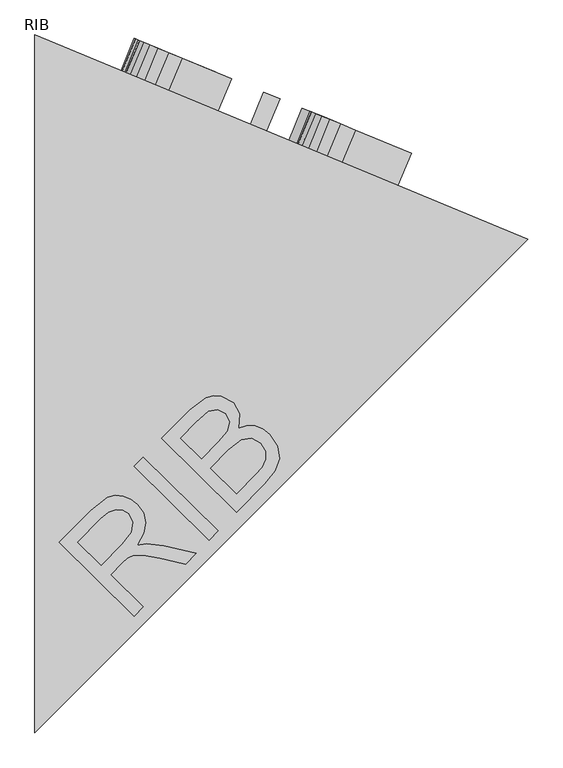
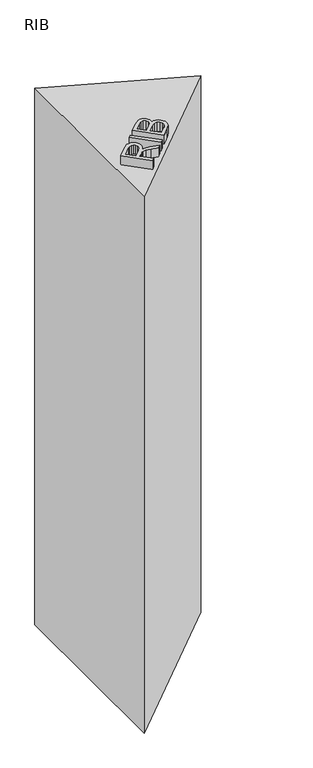
"""IFC4 building model written with IfcOpenShell, lengths in millimetres: geographic element geometry, NO_Origo : RIB."""

from ifc_helpers import new_model, si_unit, frame, origin, origin_with_axes, place, context, project, spatial, polyline, outline, extrude, source, transform, mapped, element, save


def rib_79407f03(model_context):
    return source(origin(), model_context, "Body", "SweptSolid", [
        extrude(outline(polyline([(0.0, 1000.0), (707.1067812, 707.1067812), (0.0, 0.0), (0.0, 1000.0)])), origin_with_axes(), (0.0, 0.0, 1.0), 3000.0),
        extrude(outline(polyline([(25.1140775, 0.0), (25.1140775, -200.9126203), (-61.4608186, -200.9126203), (-84.7293549, -199.5575883), (-101.658058, -195.4924922), (-114.0311558, -187.9876995), (-123.6328759, -176.3135776), (-129.7948993, -161.837421), (-131.8489071, -145.9265248), (-128.4459986, -126.1344734), (-118.2372733, -109.7269364), (-100.9161627, -97.6971952), (-76.1760985, -91.0385311), (-90.4499198, -80.2963768), (-110.806057, -54.4465353), (-144.307844, 0.0), (-115.1225391, 0.0), (-88.9783919, -41.6442419), (-70.0937828, -69.210866), (-56.8255055, -82.2338887), (-44.8816034, -87.0163546), (-30.3134764, -87.8992714), (0.0, -87.8992714), (0.0, 0.0), (25.1140775, 0.0)]), holes=[polyline([(0.0, -113.0133489), (-56.2123689, -113.0133489), (-84.882639, -116.5695415), (-94.3126808, -121.1925919), (-101.1675487, -127.9493579), (-106.7348295, -144.994557), (-104.0799478, -157.2450275), (-96.1153027, -167.1165277), (-82.4116983, -173.628039), (-62.5399392, -175.7985428), (0.0, -175.7985428), (0.0, -113.0133489)])]), frame((497.5715471, 793.899117, 2400.0), z_axis=(0.38268343236508784, 0.9238795325112875, 0.0), x_axis=(0.9238795325112875, -0.38268343236508784, 0.0)), (0.0, 0.0, 1.0), 50.0),
        extrude(outline(polyline([(328.1863632, 918.1803674), (351.3887454, 908.569626), (332.2545738, 862.3756494), (309.0521916, 871.9863908), (328.1863632, 918.1803674)])), frame((0.0, 0.0, 2400.0), z_axis=(0.0, 0.0, 1.0), x_axis=(1.0, 0.0, 0.0)), (0.0, 0.0, 1.0), 200.9126203),
        extrude(outline(polyline([(76.0779965, 0.0), (76.0779965, -200.9126203), (-0.5886112, -200.9126203), (-21.6743809, -199.434961), (-38.1371002, -195.0019829), (-50.7554526, -187.5033216), (-60.3081217, -176.8286123), (-66.3229924, -164.2715736), (-68.3279493, -151.1259236), (-66.6418234, -139.0287373), (-61.583446, -127.6550523), (-53.1160287, -117.7038444), (-41.2027834, -109.8740892), (-55.4336854, -102.4428729), (-65.948979, -91.1366329), (-72.4420962, -76.703396), (-74.6064686, -59.8911888), (-68.6958312, -32.8886504), (-54.0541278, -13.6606848), (-32.2019373, -3.4580908), (0.0, 0.0), (76.0779965, 0.0)]), holes=[polyline([(50.9639191, -119.2918683), (5.101297, -119.2918683), (-21.6805123, -121.4501093), (-37.7937437, -130.7452611), (-43.2138717, -147.1037471), (-38.1616256, -163.4867587), (-23.6916005, -173.1743179), (8.5839132, -175.7985428), (50.9639191, -175.7985428), (50.9639191, -119.2918683)]), polyline([(50.9639191, -25.1140775), (-0.5395603, -25.1140775), (-19.1789147, -26.0950962), (-34.9487895, -31.5642752), (-45.3966382, -42.7233624), (-49.4923911, -59.6459342), (-44.6853997, -79.1682054), (-38.3884862, -86.2254083), (-29.1117286, -90.8178019), (1.9129864, -94.1777908), (50.9639191, -94.1777908), (50.9639191, -25.1140775)])]), frame((192.3605232, 920.3216624, 2400.0), z_axis=(0.38268343236508784, 0.9238795325112875, 0.0), x_axis=(0.9238795325112875, -0.38268343236508784, 0.0)), (0.0, 0.0, 1.0), 50.0),
        extrude(outline(polyline([(142.0846737, 166.9156415), (34.8288922, 272.7551681), (80.4360125, 318.9725642), (104.5051668, 337.5762862), (115.0296187, 340.2280985), (126.319893, 339.2040535), (137.2940026, 334.8676564), (146.8699607, 327.5824121), (155.6431762, 315.3394631), (159.0243303, 301.2462182), (156.3216686, 285.6622725), (146.8434364, 268.9472211), (160.0974204, 270.9082992), (184.6206627, 268.1577423), (231.3350949, 257.3603361), (215.9604566, 241.7799674), (179.9563975, 249.7610286), (155.2918548, 254.2015408), (141.3499598, 253.9788127), (132.5049003, 250.1220185), (124.3591622, 242.810042), (108.3902102, 226.627407), (155.3146145, 180.3226141), (142.0846737, 166.9156415)]), holes=[polyline([(94.9832375, 239.8573479), (124.595566, 269.8659235), (137.8004388, 287.0447247), (140.3041941, 301.7331255), (134.1375442, 313.6844846), (126.1991419, 318.7206668), (116.7335855, 319.6690426), (106.0384872, 315.7836943), (94.4114592, 306.3187042), (61.4658058, 272.9322), (94.9832375, 239.8573479)])]), frame((0.0, 0.0, 3000.0), z_axis=(0.0, 0.0, 1.0), x_axis=(1.0, 0.0, 0.0)), (0.0, 0.0, 1.0), 50.0),
        extrude(outline(polyline([(249.577943, 275.8472945), (142.3221615, 381.6868212), (155.5521023, 395.0937938), (262.8078838, 289.2542672), (249.577943, 275.8472945)])), frame((0.0, 0.0, 3000.0), z_axis=(0.0, 0.0, 1.0), x_axis=(1.0, 0.0, 0.0)), (0.0, 0.0, 1.0), 50.0),
        extrude(outline(polyline([(289.2677655, 316.0682125), (182.011984, 421.9077392), (222.3994792, 462.8356656), (245.3351431, 479.7669736), (255.9855205, 482.5529434), (266.7164256, 482.0291974), (284.6624197, 472.770508), (293.6392157, 456.8056927), (292.3950501, 436.5587187), (303.8589035, 440.2410662), (315.4340515, 439.898524), (326.559667, 435.7614887), (336.6749229, 428.0603568), (347.9763498, 410.6802344), (350.5279044, 392.7346911), (344.4628882, 375.6943903), (329.3451839, 356.681913), (289.2677655, 316.0682125)]), holes=[polyline([(238.8145861, 392.3174042), (262.9747319, 416.8008406), (275.9310618, 432.2350681), (279.4572615, 445.7336312), (273.5796894, 457.2446776), (262.1722425, 463.178041), (249.3778877, 460.5566667), (230.9744227, 444.7090375), (208.6488975, 422.0847711), (238.8145861, 392.3174042)]), polyline([(289.0907336, 342.7051261), (316.2224482, 370.1998943), (325.5178351, 380.6671764), (330.9056251, 391.9669422), (330.4522875, 403.4229905), (323.5759095, 414.5241854), (310.6217897, 422.2422189), (296.1986213, 420.0652601), (278.0612869, 405.2729569), (252.2215587, 379.0874633), (289.0907336, 342.7051261)])]), frame((0.0, 0.0, 3000.0), z_axis=(0.0, 0.0, 1.0), x_axis=(1.0, 0.0, 0.0)), (0.0, 0.0, 1.0), 50.0),
    ])


if __name__ == "__main__":
    model = new_model("IFC4")
    model_context = context("Model", 3, world=origin())
    ifc_project = project(units=[si_unit("LENGTHUNIT", "METRE", prefix="MILLI")], contexts=[model_context])
    site = spatial("IfcSite", under=ifc_project)
    building = spatial("IfcBuilding", under=site)
    placement = place(None, origin())
    rib_shape = rib_79407f03(model_context)
    element("IfcGeographicElement", 1, ObjectType="NO_Origo : RIB", at=placement, inside=building, context=model_context, shape_type="MappedRepresentation", body=[
        mapped(rib_shape, transform((0.0, 0.0, 0.0), x_axis=(1.0, 0.0, 0.0), y_axis=(0.0, 1.0, 0.0), z_axis=(0.0, 0.0, 1.0))),
    ])
    save(model, "model.ifc")

# Revit data of these elements
# Type "NO_Origo : RIB"
#   Manufacturer = "Norconsult"
#   Text Height = 400 mm
#   Sill Height = 0 mm
#   Height3 = 1000 mm
#   Height = 3000 mm
#   SITE = no
#   RIVv = no
#   RIVr = no
#   RIV = no
#   RISt = no
#   RIPre = no
#   RIMEK = no
#   RIG = no
#   RIE = no
#   RIBr = no
#   RIB = yes
#   LARK = no
#   ARK = no
#   Top Material = none
#   Material = none
#   Assembly Code = ""
# Element 1 (IfcGeographicElement, "NO_Origo : RIB")
#   Materials on its faces: "RIB"
# Materials
#   "RIB": class "Unassigned", colour RGB 0 255 0, transparency 0, Description = "Dummy material", Cost = 0
